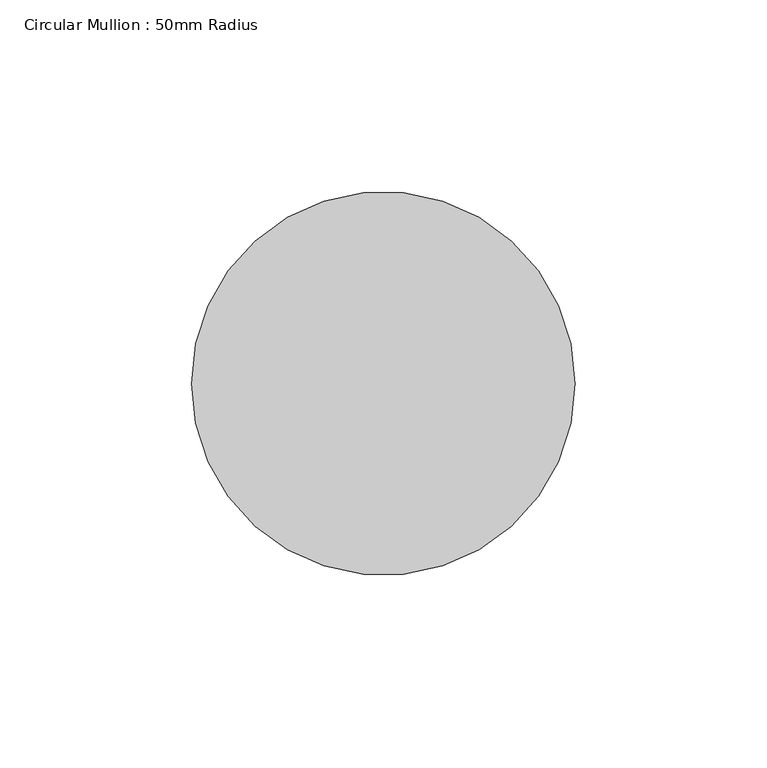
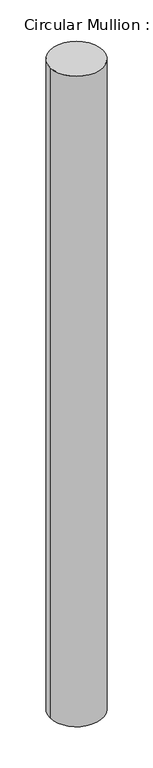
"""IFC4 building model written with IfcOpenShell, lengths in millimetres: member geometry, Circular Mullion : 50mm Radius."""

from ifc_helpers import new_model, si_unit, point, frame, origin, origin_2d, place, context, project, spatial, circle_curve, trimmed, segment, composite_curve, outline, extrude, source, transform, mapped, element, save


def circular_mullion_50mm_radius_b6626e89(model_context):
    return source(origin(), model_context, "Body", "SweptSolid", [
        extrude(outline(composite_curve([segment(trimmed(circle_curve(origin_2d(), 50.0), [point((50.0, 0.0))], [point((-50.0, 0.0))], False, "CARTESIAN"), True, "CONTINUOUS"), segment(trimmed(circle_curve(origin_2d(), 50.0), [point((-50.0, 0.0))], [point((50.0, 0.0))], False, "CARTESIAN"), True, "CONTINUOUS")], self_intersect=False)), frame((0.0, 0.0, -1299.2526078), z_axis=(0.0, 0.0, 1.0), x_axis=(1.0, 0.0, 0.0)), (0.0, 0.0, 1.0), 1299.2526078),
    ])


if __name__ == "__main__":
    model = new_model("IFC4")
    model_context = context("Model", 3, world=origin())
    ifc_project = project(units=[si_unit("LENGTHUNIT", "METRE", prefix="MILLI")], contexts=[model_context])
    site = spatial("IfcSite", under=ifc_project)
    building = spatial("IfcBuilding", under=site)
    placement = place(None, origin())
    circular_mullion_50mm_radius_shape = circular_mullion_50mm_radius_b6626e89(model_context)
    element("IfcMember", 1, ObjectType="Circular Mullion : 50mm Radius", at=placement, inside=building, context=model_context, shape_type="MappedRepresentation", body=[
        mapped(circular_mullion_50mm_radius_shape, transform((0.0, 0.0, 0.0), x_axis=(1.0, 0.0, 0.0), y_axis=(0.0, 1.0, 0.0), z_axis=(0.0, 0.0, 1.0))),
    ])
    save(model, "model.ifc")

# Revit data of these elements
# Type "Circular Mullion : 50mm Radius"
#   built-in parameter 1007350 = 0.164042 (stored number, unit not read)
# Element 1 (IfcMember, "Circular Mullion : 50mm Radius")
#   Materials on its faces: "Aluminium"
# Materials
#   "Aluminium": class "Metal", colour RGB 247 247 247, transparency 0, Description = "Aluminium 6061", Cost = 0
